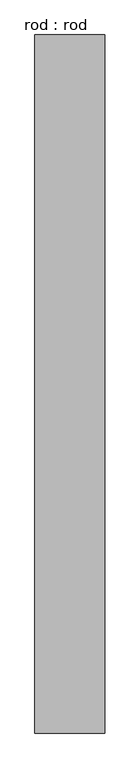
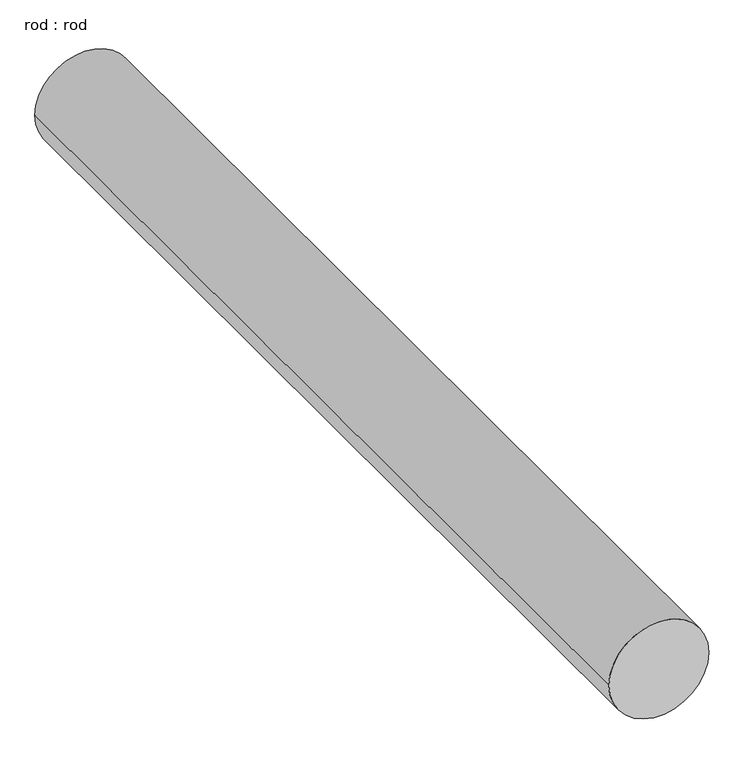
"""IFC4 building model written with IfcOpenShell, lengths in millimetres: proxy geometry, rod : rod."""

from ifc_helpers import new_model, si_unit, point, frame, frame_2d, origin, place, context, project, spatial, circle_curve, trimmed, segment, composite_curve, outline, extrude, source, transform, mapped, element, save


def rod_rod_e8063014(model_context):
    return source(origin(), model_context, "Body", "SweptSolid", [
        extrude(outline(composite_curve([segment(trimmed(circle_curve(frame_2d((0.0108462, 0.0)), 200.0), [point((0.0108462, 200.0))], [point((0.0108462, -200.0))], False, "CARTESIAN"), True, "CONTINUOUS"), segment(trimmed(circle_curve(frame_2d((0.0108462, 0.0)), 200.0), [point((0.0108462, -200.0))], [point((0.0108462, 200.0))], False, "CARTESIAN"), True, "CONTINUOUS")], self_intersect=False)), frame((0.0, 2099.0495414, 0.0), z_axis=(0.0, 1.0, 0.0), x_axis=(0.0, 0.0, 1.0)), (0.0, 0.0, 1.0), 3987.3581479),
    ])


if __name__ == "__main__":
    model = new_model("IFC4")
    model_context = context("Model", 3, world=origin())
    ifc_project = project(units=[si_unit("LENGTHUNIT", "METRE", prefix="MILLI")], contexts=[model_context])
    site = spatial("IfcSite", under=ifc_project)
    building = spatial("IfcBuilding", under=site)
    placement = place(None, origin())
    rod_rod_shape = rod_rod_e8063014(model_context)
    element("IfcBuildingElementProxy", 1, Name="rod : rod", ObjectType="rod : rod", at=placement, inside=building, context=model_context, shape_type="MappedRepresentation", body=[
        mapped(rod_rod_shape, transform((0.0, 0.0, 0.0), x_axis=(1.0, 0.0, 0.0), y_axis=(0.0, 1.0, 0.0), z_axis=(0.0, 0.0, 1.0))),
    ])
    save(model, "model.ifc")

# Revit data of these elements
# Type "rod : rod"
#   Default Elevation = 0
